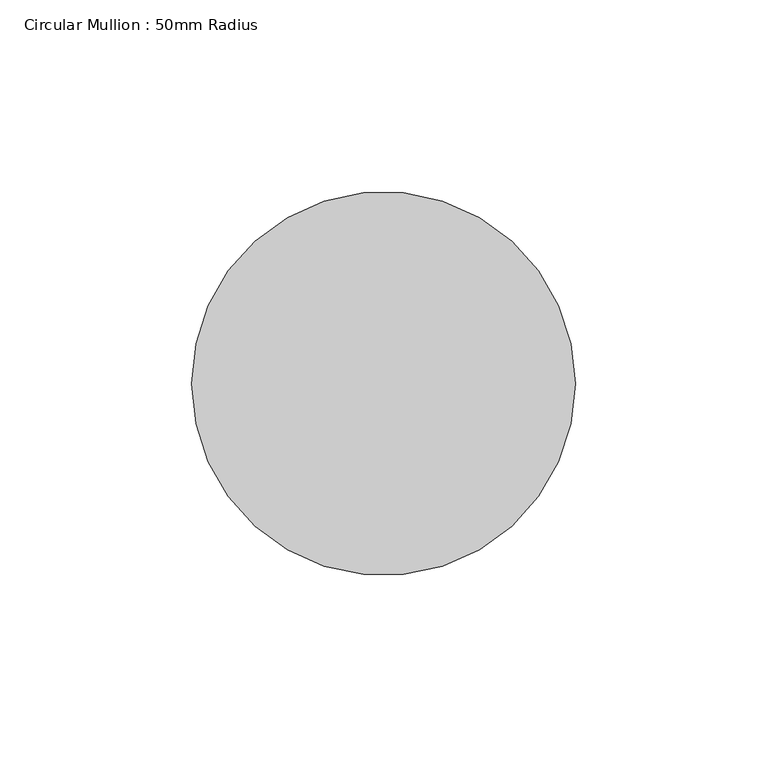
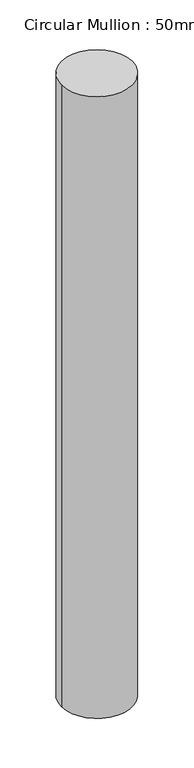
"""IFC4 building model written with IfcOpenShell, lengths in millimetres: member geometry, Circular Mullion : 50mm Radius."""

import ifcopenshell
import ifcopenshell.guid

model = None  # the IFC model being written
_history = None  # IfcOwnerHistory: only IFC2X3 demands one
_inside = {}  # id of a spatial element -> (the spatial element, [elements in it])
_under = {}  # id of a project, library or spatial element -> (it, [spatial elements below it])
_declared = {}  # id of a project -> (the project, [libraries it declares])
_typed = {}  # id of a type object -> (the type object, [elements of that type])
_made_of = {}  # id of a material, layer set ... -> (it, [elements and type objects made of it])


def new_model(schema):
    """Start an empty IFC model of exactly this schema.

    Asked for "IFC4X3", IfcOpenShell would pick the latest addendum, in which some entities
    have other attributes; the version numbers below select the first issue.
    IFC2X3 requires an IfcOwnerHistory on every rooted entity: one is made here for all.
    """
    global model, _history
    if schema == "IFC4X3":
        model = ifcopenshell.file(schema_version=(4, 3, 0, 0))
    else:
        model = ifcopenshell.file(schema=schema)
    _inside.clear()
    _under.clear()
    _declared.clear()
    _typed.clear()
    _made_of.clear()
    _history = None
    if model.schema == "IFC2X3":
        org = make("IfcOrganization", Name="unknown")
        user = make(
            "IfcPersonAndOrganization",
            ThePerson=make("IfcPerson", FamilyName="unknown"),
            TheOrganization=org,
        )
        app = make(
            "IfcApplication",
            ApplicationDeveloper=org,
            Version="unknown",
            ApplicationFullName="unknown",
            ApplicationIdentifier="unknown",
        )
        _history = make(
            "IfcOwnerHistory",
            OwningUser=user,
            OwningApplication=app,
            ChangeAction="ADDED",
            CreationDate=0,
        )
    return model


def make(cls, **values):
    """One entity of the class cls with the attributes given. An attribute that is None is left unset."""
    return model.create_entity(
        cls, **{name: value for name, value in values.items() if value is not None}
    )


def rooted(cls, **values):
    """An entity with a GlobalId (a new one), such as an element, a storey or a relation."""
    return make(cls, GlobalId=ifcopenshell.guid.new(), OwnerHistory=_history, **values)


def si_unit(unit_type, name, prefix=None):
    """IfcSIUnit, for example si_unit("LENGTHUNIT", "METRE", prefix="MILLI")."""
    return make("IfcSIUnit", UnitType=unit_type, Prefix=prefix, Name=name)


def assignment(units):
    """IfcUnitAssignment: the units of a project."""
    return None if units is None else make("IfcUnitAssignment", Units=units)


def point(xyz):
    """IfcCartesianPoint."""
    return None if xyz is None else make("IfcCartesianPoint", Coordinates=xyz)


def direction(xyz):
    """IfcDirection."""
    return None if xyz is None else make("IfcDirection", DirectionRatios=xyz)


def frame(location, z_axis=None, x_axis=None):
    """IfcAxis2Placement3D, a coordinate frame: its origin and axes. An axis left out is left unset."""
    return make(
        "IfcAxis2Placement3D",
        Location=point(location),
        Axis=direction(z_axis),
        RefDirection=direction(x_axis),
    )


def frame_2d(location, x_axis=None):
    """IfcAxis2Placement2D, a coordinate frame in the plane: its origin and x axis."""
    return make(
        "IfcAxis2Placement2D", Location=point(location), RefDirection=direction(x_axis)
    )


def origin():
    """The frame at (0, 0, 0) with its axes left unset."""
    return frame((0.0, 0.0, 0.0))


def origin_2d():
    """The frame at (0, 0) in the plane with its x axis left unset."""
    return frame_2d((0.0, 0.0))


def place(relative_to, where):
    """IfcLocalPlacement: puts the frame where relative to a parent placement (None: the world)."""
    return make(
        "IfcLocalPlacement", PlacementRelTo=relative_to, RelativePlacement=where
    )


def context(
    kind, dimensions, precision=None, world=None, true_north=None, identifier=None
):
    """IfcGeometricRepresentationContext, for example the 3D "Model" context."""
    return make(
        "IfcGeometricRepresentationContext",
        ContextIdentifier=identifier,
        ContextType=kind,
        CoordinateSpaceDimension=dimensions,
        Precision=precision,
        WorldCoordinateSystem=world,
        TrueNorth=true_north,
    )


def project(units=None, contexts=None):
    """IfcProject with its units and contexts."""
    return rooted(
        "IfcProject",
        Name="project",
        RepresentationContexts=contexts,
        UnitsInContext=assignment(units),
    )


def spatial(cls, under=None, at=None, **own):
    """A site, building, storey or space (cls), placed at a placement, below another one or the project."""
    s = rooted(cls, ObjectPlacement=at, **own)
    if under is not None:
        _under.setdefault(under.id(), (under, []))[1].append(s)
    return s


def circle_curve(where, radius):
    """IfcCircle in the frame where."""
    return make("IfcCircle", Position=where, Radius=radius)


def trimmed(basis, trim1, trim2, sense, master):
    """IfcTrimmedCurve: the piece of a basis curve between two trims."""
    return make(
        "IfcTrimmedCurve",
        BasisCurve=basis,
        Trim1=trim1,
        Trim2=trim2,
        SenseAgreement=sense,
        MasterRepresentation=master,
    )


def segment(curve, same_sense, transition):
    """IfcCompositeCurveSegment."""
    return make(
        "IfcCompositeCurveSegment",
        Transition=transition,
        SameSense=same_sense,
        ParentCurve=curve,
    )


def composite_curve(segments, self_intersect=None):
    """IfcCompositeCurve: segments joined end to end."""
    return make("IfcCompositeCurve", Segments=segments, SelfIntersect=self_intersect)


def outline(outer, holes=None, kind="AREA"):
    """IfcArbitraryClosedProfileDef: a profile drawn as a closed curve; with holes, ...WithVoids."""
    if holes is None:
        return make("IfcArbitraryClosedProfileDef", ProfileType=kind, OuterCurve=outer)
    return make(
        "IfcArbitraryProfileDefWithVoids",
        ProfileType=kind,
        OuterCurve=outer,
        InnerCurves=holes,
    )


def extrude(swept, where, along, depth):
    """IfcExtrudedAreaSolid: the profile swept, set in the frame where, extruded along a direction by depth."""
    return make(
        "IfcExtrudedAreaSolid",
        SweptArea=swept,
        Position=where,
        ExtrudedDirection=direction(along),
        Depth=depth,
    )


def shape(context_of_items, identifier, shape_type, items):
    """IfcShapeRepresentation: the items that make up one representation, for example the "Body"."""
    return make(
        "IfcShapeRepresentation",
        ContextOfItems=context_of_items,
        RepresentationIdentifier=identifier,
        RepresentationType=shape_type,
        Items=items,
    )


def source(mapping_origin, context_of_items, identifier, shape_type, items):
    """IfcRepresentationMap: a shape defined once, which mapped items show again and again."""
    return make(
        "IfcRepresentationMap",
        MappingOrigin=mapping_origin,
        MappedRepresentation=shape(context_of_items, identifier, shape_type, items),
    )


def transform(
    local_origin,
    x_axis=None,
    y_axis=None,
    z_axis=None,
    scale=None,
    scale2=None,
    scale3=None,
    uniform=True,
):
    """IfcCartesianTransformationOperator3D, or its non-uniform kind. x_axis, y_axis, z_axis: its Axis1, 2, 3."""
    if uniform:
        return make(
            "IfcCartesianTransformationOperator3D",
            Axis1=direction(x_axis),
            Axis2=direction(y_axis),
            LocalOrigin=point(local_origin),
            Scale=scale,
            Axis3=direction(z_axis),
        )
    return make(
        "IfcCartesianTransformationOperator3DnonUniform",
        Axis1=direction(x_axis),
        Axis2=direction(y_axis),
        LocalOrigin=point(local_origin),
        Scale=scale,
        Axis3=direction(z_axis),
        Scale2=scale2,
        Scale3=scale3,
    )


def mapped(mapping_source, mapping_target):
    """IfcMappedItem: shows the shape of a source again, moved by a transform."""
    return make(
        "IfcMappedItem", MappingSource=mapping_source, MappingTarget=mapping_target
    )


def made_of(thing, what):
    """Note that an element or type object is made of a material, layer set ...; save() writes the relation."""
    if what is not None:
        _made_of.setdefault(what.id(), (what, []))[1].append(thing)
    return thing


def element(
    cls,
    number,
    at=None,
    inside=None,
    cuts=None,
    type_object=None,
    material=None,
    context=None,
    identifier="Body",
    shape_type=None,
    held_by="IfcProductDefinitionShape",
    body=None,
    shapes=None,
    **own,
):
    """One element of the class cls, such as IfcWall. Its Tag is "e" and its number.

    at: its placement. inside: the storey or other place that contains it. cuts: it is an
    opening in that element (IfcRelVoidsElement). A single representation is given by context,
    identifier, shape_type and body (its items); several are given by shapes. held_by: the class
    of the entity that holds the representations. save() writes the other relations.
    """
    e = rooted(cls, Tag="e%d" % number, ObjectPlacement=at, **own)
    if body is not None:
        shapes = [shape(context, identifier, shape_type, body)]
    if shapes is not None:
        e.Representation = make(held_by, Representations=shapes)
    if inside is not None:
        _inside.setdefault(inside.id(), (inside, []))[1].append(e)
    if cuts is not None:
        rooted(
            "IfcRelVoidsElement", RelatingBuildingElement=cuts, RelatedOpeningElement=e
        )
    if type_object is not None:
        _typed.setdefault(type_object.id(), (type_object, []))[1].append(e)
    return made_of(e, material)


def aggregate(whole, parts):
    """IfcRelAggregates: a whole, such as a stair, and the parts it consists of."""
    return rooted("IfcRelAggregates", RelatingObject=whole, RelatedObjects=parts)


def save(model, path):
    """Write the relations noted so far, then the file.

    IfcRelAggregates (storeys below a building ...), IfcRelContainedInSpatialStructure (elements
    in a storey), IfcRelDefinesByType, IfcRelAssociatesMaterial and IfcRelDeclares: one each for
    every whole, place, type object, material and project.
    """
    for whole, parts in _under.values():
        aggregate(whole, parts)
    for where, things in _inside.values():
        rooted(
            "IfcRelContainedInSpatialStructure",
            RelatedElements=things,
            RelatingStructure=where,
        )
    for kind, things in _typed.values():
        rooted("IfcRelDefinesByType", RelatedObjects=things, RelatingType=kind)
    for what, things in _made_of.values():
        rooted("IfcRelAssociatesMaterial", RelatedObjects=things, RelatingMaterial=what)
    for by, libraries in _declared.values():
        rooted("IfcRelDeclares", RelatingContext=by, RelatedDefinitions=libraries)
    model.write(path)


def circular_mullion_50mm_radius_8efff23f(model_context):
    return source(origin(), model_context, "Body", "SweptSolid", [
        extrude(outline(composite_curve([segment(trimmed(circle_curve(origin_2d(), 50.0), [point((50.0, 0.0))], [point((-50.0, 0.0))], False, "CARTESIAN"), True, "CONTINUOUS"), segment(trimmed(circle_curve(origin_2d(), 50.0), [point((-50.0, 0.0))], [point((50.0, 0.0))], False, "CARTESIAN"), True, "CONTINUOUS")], self_intersect=False)), frame((0.0, 0.0, -925.4290944), z_axis=(0.0, 0.0, 1.0), x_axis=(1.0, 0.0, 0.0)), (0.0, 0.0, 1.0), 925.4290944),
    ])


if __name__ == "__main__":
    model = new_model("IFC4")
    model_context = context("Model", 3, world=origin())
    ifc_project = project(units=[si_unit("LENGTHUNIT", "METRE", prefix="MILLI")], contexts=[model_context])
    site = spatial("IfcSite", under=ifc_project)
    building = spatial("IfcBuilding", under=site)
    placement = place(None, origin())
    circular_mullion_50mm_radius_shape = circular_mullion_50mm_radius_8efff23f(model_context)
    element("IfcMember", 1, ObjectType="Circular Mullion : 50mm Radius", at=placement, inside=building, context=model_context, shape_type="MappedRepresentation", body=[
        mapped(circular_mullion_50mm_radius_shape, transform((0.0, 0.0, 0.0), x_axis=(1.0, 0.0, 0.0), y_axis=(0.0, 1.0, 0.0), z_axis=(0.0, 0.0, 1.0))),
    ])
    save(model, "model.ifc")

# Revit data of these elements
# Type "Circular Mullion : 50mm Radius"
#   built-in parameter 1007350 = 0.164042 (stored number, unit not read)
# Element 1 (IfcMember, "Circular Mullion : 50mm Radius")
#   Materials on its faces: "Aluminium"
# Materials
#   "Aluminium": class "Metal", colour RGB 247 247 247, transparency 0, Description = "Aluminium 6061", Cost = 0
